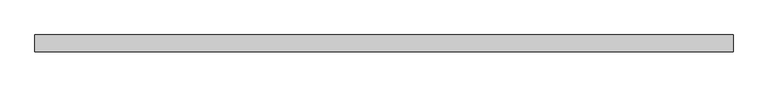
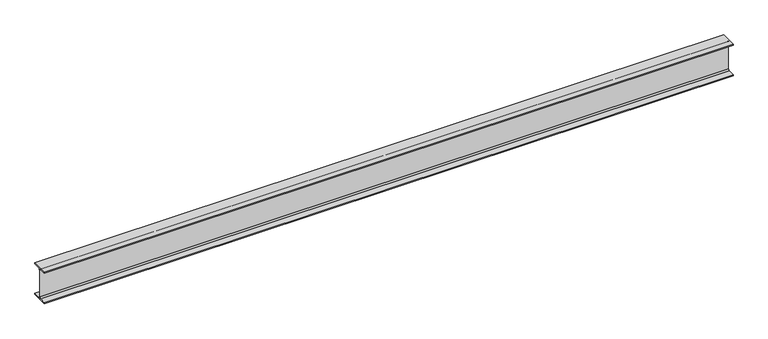
"""IFC4 building model written with IfcOpenShell, lengths in millimetres: beam geometry, 0912_Steel Framing_H-KSD3502 : H_SB_ASB_H-400x200x8x13."""

from ifc_helpers import new_model, si_unit, point, frame, frame_2d, origin, place, context, project, spatial, polyline, circle_curve, trimmed, segment, composite_curve, outline, extrude, source, transform, mapped, element, save


def beam_a7978027(model_context):
    return source(origin(), model_context, "Body", "SweptSolid", [
        extrude(outline(composite_curve([segment(polyline([(100.0, -187.0), (100.0, -200.0), (-100.0, -200.0), (-100.0, -187.0), (-20.0, -187.0)]), True, "CONTINUOUS"), segment(trimmed(circle_curve(frame_2d((-20.0, -171.0)), 16.0), [point((-20.0, -187.0))], [point((-4.0, -171.0))], True, "CARTESIAN"), True, "CONTINUOUS"), segment(polyline([(-4.0, -171.0), (-4.0, 171.0)]), True, "CONTINUOUS"), segment(trimmed(circle_curve(frame_2d((-20.0, 171.0)), 16.0), [point((-4.0, 171.0))], [point((-20.0, 187.0))], True, "CARTESIAN"), True, "CONTINUOUS"), segment(polyline([(-20.0, 187.0), (-100.0, 187.0), (-100.0, 200.0), (100.0, 200.0), (100.0, 187.0), (20.0, 187.0)]), True, "CONTINUOUS"), segment(trimmed(circle_curve(frame_2d((20.0, 171.0)), 16.0), [point((20.0, 187.0))], [point((4.0, 171.0))], True, "CARTESIAN"), True, "CONTINUOUS"), segment(polyline([(4.0, 171.0), (4.0, -171.0)]), True, "CONTINUOUS"), segment(trimmed(circle_curve(frame_2d((20.0, -171.0)), 16.0), [point((4.0, -171.0))], [point((20.0, -187.0))], True, "CARTESIAN"), True, "CONTINUOUS"), segment(polyline([(20.0, -187.0), (100.0, -187.0)]), True, "CONTINUOUS")], self_intersect=False)), frame((-4154.8, 0.0, 0.0), z_axis=(1.0, 0.0, 0.0), x_axis=(0.0, 1.0, 0.0)), (0.0, 0.0, 1.0), 8309.6),
    ])


if __name__ == "__main__":
    model = new_model("IFC4")
    model_context = context("Model", 3, world=origin())
    ifc_project = project(units=[si_unit("LENGTHUNIT", "METRE", prefix="MILLI")], contexts=[model_context])
    site = spatial("IfcSite", under=ifc_project)
    building = spatial("IfcBuilding", under=site)
    placement = place(None, origin())
    beam_shape = beam_a7978027(model_context)
    element("IfcBeam", 1, ObjectType="0912_Steel Framing_H-KSD3502 : H_SB_ASB_H-400x200x8x13", at=placement, inside=building, context=model_context, shape_type="MappedRepresentation", body=[
        mapped(beam_shape, transform((0.0, 0.0, 0.0), x_axis=(1.0, 0.0, 0.0), y_axis=(0.0, 1.0, 0.0), z_axis=(0.0, 0.0, 1.0))),
    ])
    save(model, "model.ifc")

# Revit data of these elements
# Type "0912_Steel Framing_H-KSD3502 : H_SB_ASB_H-400x200x8x13"
#   H_WM Code_1 = "S01AA002-00001 | Main Steel Structure Fabrication Work | Shelter/Building | Medium Steel - Standard (90KG/M>Weight≥30KG/M) | Material: (   )"
#   H_WM Code_2 = "S03AA028-00001 | Main Steel Structure Erection Work | Shelter/Building | Medium Steel (90KG/M>Weight≥30KG/M) | Material: (   )"
#   H_WM Code_3 = "S01AA010-00001 | Main Steel Structure Fabrication Work | Shelter/Building | Steel Painting/Coating | for Non-Fireproofed Steel Surface, Surface Preparation, Primer, Second & Final Coat | Material: (   )"
#   H_Q'ty Cal Type Tag = "SB-Q2"
#   Width = 20.0 cm
#   Web Thickness = 0.8 cm
#   Web Fillet = 1.6 cm
#   Warping Constant = 649000.0 cm⁶
#   W = 0
#   Torsional Moment of Inertia = 35.8981 cm⁴
#   Section Area = 84.12 cm²
#   Plastic Modulus weak axis = 268.0 cm³
#   Plastic Modulus strong axis = 1330.0 cm³
#   Perimeter = 1.56 m²/m
#   Nominal Weight = 66.00 kgf/m
#   Moment of Inertia weak axis = 1740.00 cm⁴
#   Moment of Inertia strong axis = 23700.00 cm⁴
#   Height = 40.0 cm
#   Flange Thickness = 1.3 cm
#   Elastic Modulus weak axis = 174.0 cm³
#   Elastic Modulus strong axis = 1190.0 cm³
#   Centroid Vertical = 20.0 cm
#   Centroid Horizontal = 10.0 cm
#   Ix = 237000000
#   Length [instance default] = 1.5240 m
#   Zx = 1330000
#   b = 0.2000 m
#   h = 0.4000 m
#   r = 0.0160 m
#   s = 0.0080 m
#   t = 0.0130 m
#   A = 0.008412 m²
#   Structural Material [instance default] = Steel, 45-345
#   Assembly Code = ""
# Element 1 (IfcBeam, "0912_Steel Framing_H-KSD3502 : H_SB_ASB_H-400x200x8x13")
#   Structural Material = none
# Materials
#   "Steel, 45-345": class "Metal", colour RGB 189 187 185, transparency 0, Description = "Steel 345 MPa", Cost = 0
